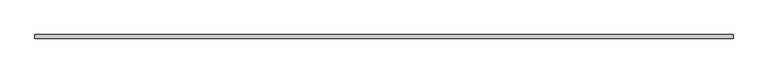
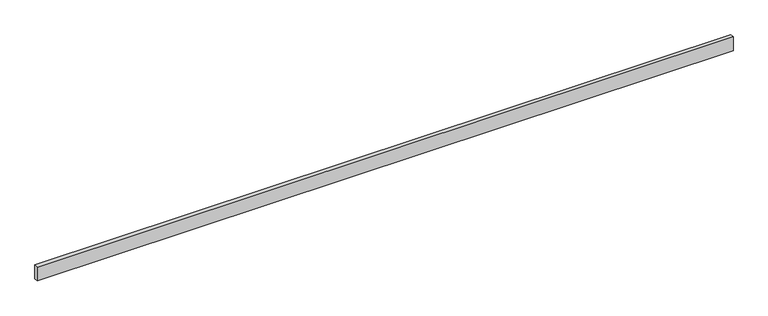
"""IFC4 building model written with IfcOpenShell, lengths in millimetres: proxy geometry, Generic Models 7:Generic Models 1:337419:Generic Models 1:337419 : Generic Models 7:Generic Models 1:337419:16 : Generic Models 7:Generic Models 1:337419:Generic Models 1:337419 : Generic Models 7:Generic Models 1:337419:301336."""

from ifc_helpers import new_model, si_unit, frame, origin, place, context, project, spatial, polyline, outline, extrude, source, transform, mapped, element, save


def generic_models_8f38601e(model_context):
    return source(origin(), model_context, "Body", "SweptSolid", [
        extrude(outline(polyline([(596182.8367242, -536531.8913358), (596182.8367242, -536557.2913358), (591306.0367242, -536557.2913358), (591306.0367242, -536531.8913358), (596182.8367242, -536531.8913358)])), frame((0.0, 0.0, 8495.1417603), z_axis=(0.0, 0.0, 1.0), x_axis=(1.0, 0.0, 0.0)), (0.0, 0.0, 1.0), 101.6),
    ])


if __name__ == "__main__":
    model = new_model("IFC4")
    model_context = context("Model", 3, world=origin())
    ifc_project = project(units=[si_unit("LENGTHUNIT", "METRE", prefix="MILLI")], contexts=[model_context])
    site = spatial("IfcSite", under=ifc_project)
    building = spatial("IfcBuilding", under=site)
    placement = place(None, origin())
    generic_models_shape = generic_models_8f38601e(model_context)
    element("IfcBuildingElementProxy", 1, Name="Generic Models 7:Generic Models 1:337419:Generic Models 1:337419 : Generic Models 7:Generic Models 1:337419:16 : Generic Models 7:Generic Models 1:337419:Generic Models 1:337419 : Generic Models 7:Generic Models 1:337419:301336", ObjectType="Generic Models 7:Generic Models 1:337419:Generic Models 1:337419 : Generic Models 7:Generic Models 1:337419:16 : Generic Models 7:Generic Models 1:337419:Generic Models 1:337419 : Generic Models 7:Generic Models 1:337419:301336", at=placement, inside=building, context=model_context, shape_type="MappedRepresentation", body=[
        mapped(generic_models_shape, transform((0.0, 0.0, 0.0), x_axis=(1.0, 0.0, 0.0), y_axis=(0.0, 1.0, 0.0), z_axis=(0.0, 0.0, 1.0))),
    ])
    save(model, "model.ifc")

# Revit data of these elements
# Type "Generic Models 7:Generic Models 1:337419:Generic Models 1:337419 : Generic Models 7:Generic Models 1:337419:16 : Generic Models 7:Generic Models 1:337419:Generic Models 1:337419 : Generic Models 7:Generic Models 1:337419:301336"
#   NameOverride = "Generic Models 7:Generic Models 1:337419:Generic Models 1:337419 : Generic Models 7:Generic Models 1:337419:301336"
#   ObjectTypeOverride = "Generic Models 1:337419 : Generic Models 7:Generic Models 1:337419"
#   Reference = "Generic Models 1"
#   Tag = "301336"
# Element 1 (IfcBuildingElementProxy, "Generic Models 7:Generic Models 1:337419:Generic Models 1:337419 : Generic Models 7:Generic Models 1:337419:16 : Generic Models 7:Generic Models 1:337419:Generic Models 1:337419 : Generic Models 7:Generic Models 1:337419:301336")
#   Materials on its faces: "1\" THERMAL SPACER @ GIRT"
# Materials
#   "1\" THERMAL SPACER @ GIRT": class "Unassigned", colour RGB 205 188 106, transparency 0, Cost = 0
